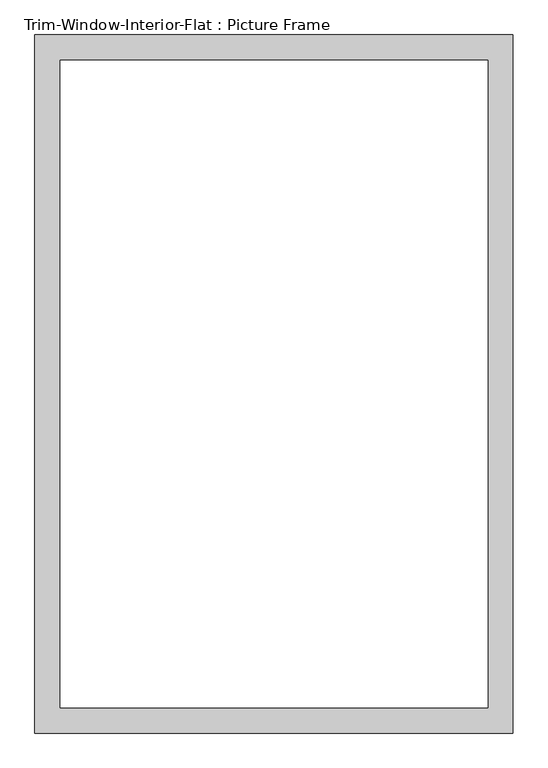
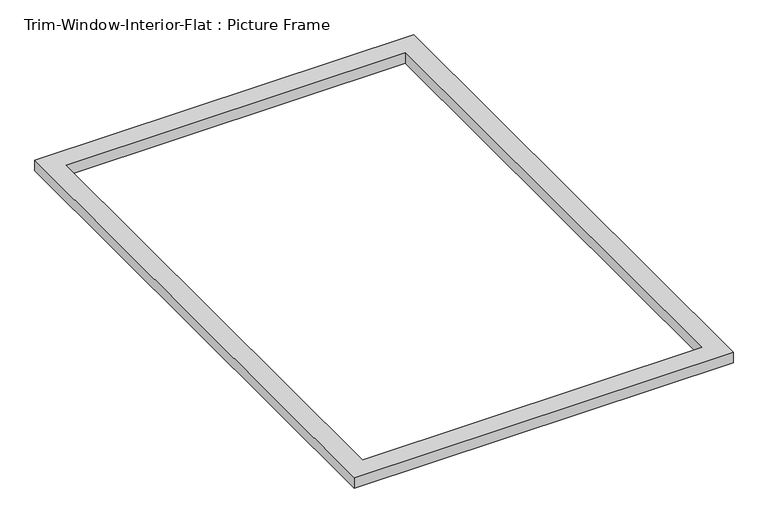
"""IFC4 building model written with IfcOpenShell, lengths in millimetres: proxy geometry, Trim-Window-Interior-Flat : Picture Frame."""

from ifc_helpers import new_model, si_unit, origin, origin_with_axes, place, context, project, spatial, polyline, outline, extrude, source, transform, mapped, element, save


def trim_window_interior_flat_picture_frame_849e6ffd(model_context):
    return source(origin(), model_context, "Body", "SweptSolid", [
        extrude(outline(polyline([(544.45, 44.45), (544.45, -1544.45), (-544.45, -1544.45), (-544.45, 44.45), (544.45, 44.45)]), holes=[polyline([(487.3, -12.7), (-487.3, -12.7), (-487.3, -1487.3), (487.3, -1487.3), (487.3, -12.7)])]), origin_with_axes(), (0.0, 0.0, 1.0), 31.75),
    ])


if __name__ == "__main__":
    model = new_model("IFC4")
    model_context = context("Model", 3, world=origin())
    ifc_project = project(units=[si_unit("LENGTHUNIT", "METRE", prefix="MILLI")], contexts=[model_context])
    site = spatial("IfcSite", under=ifc_project)
    building = spatial("IfcBuilding", under=site)
    placement = place(None, origin())
    trim_window_interior_flat_picture_frame_shape = trim_window_interior_flat_picture_frame_849e6ffd(model_context)
    element("IfcBuildingElementProxy", 1, Name="Trim-Window-Interior-Flat : Picture Frame", ObjectType="Trim-Window-Interior-Flat : Picture Frame", at=placement, inside=building, context=model_context, shape_type="MappedRepresentation", body=[
        mapped(trim_window_interior_flat_picture_frame_shape, transform((0.0, 0.0, 0.0), x_axis=(1.0, 0.0, 0.0), y_axis=(0.0, 1.0, 0.0), z_axis=(0.0, 0.0, 1.0))),
    ])
    save(model, "model.ifc")

# Revit data of these elements
# Type "Trim-Window-Interior-Flat : Picture Frame"
#   Trim Thickness_Picture Frame = 0.03175 m
#   Trim Width = 0.05715 m
#   Trim Thickness_with Sill = 0.01905 m
#   Sill Thickness = 0.03175 m
#   Opening Width [instance default] = 0.6096 m
#   Opening Height [instance default] = 0.9144 m
#   Default Elevation = 1.2192 m
#   Sill = no
#   Picture Frame = yes
#   Trim Material [instance default] = none
# Element 1 (IfcBuildingElementProxy, "Trim-Window-Interior-Flat : Picture Frame")
#   Opening Width = 1 m
#   Opening Height = 1.5 m
#   Trim Material = Wood - Stained
#   Materials on its faces: "Wood - Stained"
# Materials
#   "Wood - Stained": class "Wood", colour RGB 224 178 126, transparency 0, Cost = 0
